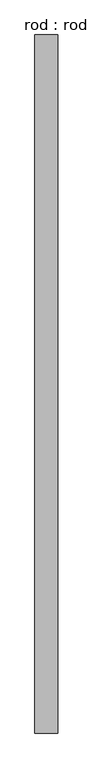
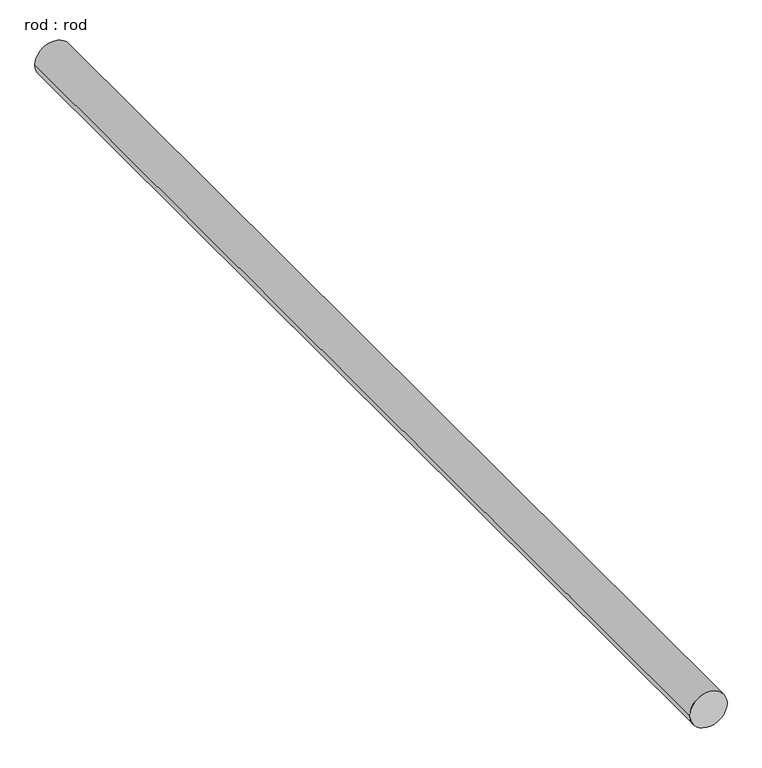
"""IFC4 building model written with IfcOpenShell, lengths in millimetres: proxy geometry, rod : rod."""

from ifc_helpers import new_model, si_unit, point, frame, frame_2d, origin, place, context, project, spatial, circle_curve, trimmed, segment, composite_curve, outline, extrude, source, transform, mapped, element, save


def rod_rod_dd8d50f1(model_context):
    return source(origin(), model_context, "Body", "SweptSolid", [
        extrude(outline(composite_curve([segment(trimmed(circle_curve(frame_2d((0.0108462, 0.0)), 200.0), [point((0.0108462, 200.0))], [point((0.0108462, -200.0))], False, "CARTESIAN"), True, "CONTINUOUS"), segment(trimmed(circle_curve(frame_2d((0.0108462, 0.0)), 200.0), [point((0.0108462, -200.0))], [point((0.0108462, 200.0))], False, "CARTESIAN"), True, "CONTINUOUS")], self_intersect=False)), frame((0.0, -2007.2713847, 0.0), z_axis=(0.0, 1.0, 0.0), x_axis=(0.0, 0.0, 1.0)), (0.0, 0.0, 1.0), 12200.0),
    ])


if __name__ == "__main__":
    model = new_model("IFC4")
    model_context = context("Model", 3, world=origin())
    ifc_project = project(units=[si_unit("LENGTHUNIT", "METRE", prefix="MILLI")], contexts=[model_context])
    site = spatial("IfcSite", under=ifc_project)
    building = spatial("IfcBuilding", under=site)
    placement = place(None, origin())
    rod_rod_shape = rod_rod_dd8d50f1(model_context)
    element("IfcBuildingElementProxy", 1, Name="rod : rod", ObjectType="rod : rod", at=placement, inside=building, context=model_context, shape_type="MappedRepresentation", body=[
        mapped(rod_rod_shape, transform((0.0, 0.0, 0.0), x_axis=(1.0, 0.0, 0.0), y_axis=(0.0, 1.0, 0.0), z_axis=(0.0, 0.0, 1.0))),
    ])
    save(model, "model.ifc")

# Revit data of these elements
# Type "rod : rod"
#   Default Elevation = 0
